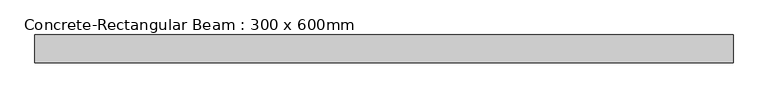
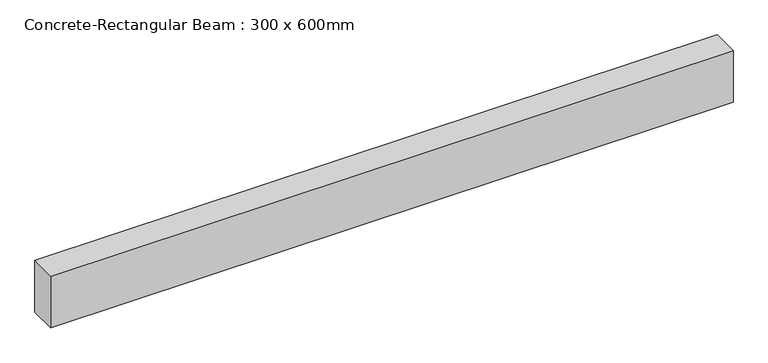
"""IFC4 building model written with IfcOpenShell, lengths in millimetres: beam geometry, Concrete-Rectangular Beam : 300 x 600mm."""

import ifcopenshell
import ifcopenshell.guid

model = None  # the IFC model being written
_history = None  # IfcOwnerHistory: only IFC2X3 demands one
_inside = {}  # id of a spatial element -> (the spatial element, [elements in it])
_under = {}  # id of a project, library or spatial element -> (it, [spatial elements below it])
_declared = {}  # id of a project -> (the project, [libraries it declares])
_typed = {}  # id of a type object -> (the type object, [elements of that type])
_made_of = {}  # id of a material, layer set ... -> (it, [elements and type objects made of it])


def new_model(schema):
    """Start an empty IFC model of exactly this schema.

    Asked for "IFC4X3", IfcOpenShell would pick the latest addendum, in which some entities
    have other attributes; the version numbers below select the first issue.
    IFC2X3 requires an IfcOwnerHistory on every rooted entity: one is made here for all.
    """
    global model, _history
    if schema == "IFC4X3":
        model = ifcopenshell.file(schema_version=(4, 3, 0, 0))
    else:
        model = ifcopenshell.file(schema=schema)
    _inside.clear()
    _under.clear()
    _declared.clear()
    _typed.clear()
    _made_of.clear()
    _history = None
    if model.schema == "IFC2X3":
        org = make("IfcOrganization", Name="unknown")
        user = make(
            "IfcPersonAndOrganization",
            ThePerson=make("IfcPerson", FamilyName="unknown"),
            TheOrganization=org,
        )
        app = make(
            "IfcApplication",
            ApplicationDeveloper=org,
            Version="unknown",
            ApplicationFullName="unknown",
            ApplicationIdentifier="unknown",
        )
        _history = make(
            "IfcOwnerHistory",
            OwningUser=user,
            OwningApplication=app,
            ChangeAction="ADDED",
            CreationDate=0,
        )
    return model


def make(cls, **values):
    """One entity of the class cls with the attributes given. An attribute that is None is left unset."""
    return model.create_entity(
        cls, **{name: value for name, value in values.items() if value is not None}
    )


def rooted(cls, **values):
    """An entity with a GlobalId (a new one), such as an element, a storey or a relation."""
    return make(cls, GlobalId=ifcopenshell.guid.new(), OwnerHistory=_history, **values)


def si_unit(unit_type, name, prefix=None):
    """IfcSIUnit, for example si_unit("LENGTHUNIT", "METRE", prefix="MILLI")."""
    return make("IfcSIUnit", UnitType=unit_type, Prefix=prefix, Name=name)


def assignment(units):
    """IfcUnitAssignment: the units of a project."""
    return None if units is None else make("IfcUnitAssignment", Units=units)


def point(xyz):
    """IfcCartesianPoint."""
    return None if xyz is None else make("IfcCartesianPoint", Coordinates=xyz)


def direction(xyz):
    """IfcDirection."""
    return None if xyz is None else make("IfcDirection", DirectionRatios=xyz)


def frame(location, z_axis=None, x_axis=None):
    """IfcAxis2Placement3D, a coordinate frame: its origin and axes. An axis left out is left unset."""
    return make(
        "IfcAxis2Placement3D",
        Location=point(location),
        Axis=direction(z_axis),
        RefDirection=direction(x_axis),
    )


def origin():
    """The frame at (0, 0, 0) with its axes left unset."""
    return frame((0.0, 0.0, 0.0))


def place(relative_to, where):
    """IfcLocalPlacement: puts the frame where relative to a parent placement (None: the world)."""
    return make(
        "IfcLocalPlacement", PlacementRelTo=relative_to, RelativePlacement=where
    )


def context(
    kind, dimensions, precision=None, world=None, true_north=None, identifier=None
):
    """IfcGeometricRepresentationContext, for example the 3D "Model" context."""
    return make(
        "IfcGeometricRepresentationContext",
        ContextIdentifier=identifier,
        ContextType=kind,
        CoordinateSpaceDimension=dimensions,
        Precision=precision,
        WorldCoordinateSystem=world,
        TrueNorth=true_north,
    )


def project(units=None, contexts=None):
    """IfcProject with its units and contexts."""
    return rooted(
        "IfcProject",
        Name="project",
        RepresentationContexts=contexts,
        UnitsInContext=assignment(units),
    )


def spatial(cls, under=None, at=None, **own):
    """A site, building, storey or space (cls), placed at a placement, below another one or the project."""
    s = rooted(cls, ObjectPlacement=at, **own)
    if under is not None:
        _under.setdefault(under.id(), (under, []))[1].append(s)
    return s


def polyline(points):
    """IfcPolyline through the points."""
    return make("IfcPolyline", Points=[point(p) for p in points])


def outline(outer, holes=None, kind="AREA"):
    """IfcArbitraryClosedProfileDef: a profile drawn as a closed curve; with holes, ...WithVoids."""
    if holes is None:
        return make("IfcArbitraryClosedProfileDef", ProfileType=kind, OuterCurve=outer)
    return make(
        "IfcArbitraryProfileDefWithVoids",
        ProfileType=kind,
        OuterCurve=outer,
        InnerCurves=holes,
    )


def extrude(swept, where, along, depth):
    """IfcExtrudedAreaSolid: the profile swept, set in the frame where, extruded along a direction by depth."""
    return make(
        "IfcExtrudedAreaSolid",
        SweptArea=swept,
        Position=where,
        ExtrudedDirection=direction(along),
        Depth=depth,
    )


def shape(context_of_items, identifier, shape_type, items):
    """IfcShapeRepresentation: the items that make up one representation, for example the "Body"."""
    return make(
        "IfcShapeRepresentation",
        ContextOfItems=context_of_items,
        RepresentationIdentifier=identifier,
        RepresentationType=shape_type,
        Items=items,
    )


def source(mapping_origin, context_of_items, identifier, shape_type, items):
    """IfcRepresentationMap: a shape defined once, which mapped items show again and again."""
    return make(
        "IfcRepresentationMap",
        MappingOrigin=mapping_origin,
        MappedRepresentation=shape(context_of_items, identifier, shape_type, items),
    )


def transform(
    local_origin,
    x_axis=None,
    y_axis=None,
    z_axis=None,
    scale=None,
    scale2=None,
    scale3=None,
    uniform=True,
):
    """IfcCartesianTransformationOperator3D, or its non-uniform kind. x_axis, y_axis, z_axis: its Axis1, 2, 3."""
    if uniform:
        return make(
            "IfcCartesianTransformationOperator3D",
            Axis1=direction(x_axis),
            Axis2=direction(y_axis),
            LocalOrigin=point(local_origin),
            Scale=scale,
            Axis3=direction(z_axis),
        )
    return make(
        "IfcCartesianTransformationOperator3DnonUniform",
        Axis1=direction(x_axis),
        Axis2=direction(y_axis),
        LocalOrigin=point(local_origin),
        Scale=scale,
        Axis3=direction(z_axis),
        Scale2=scale2,
        Scale3=scale3,
    )


def mapped(mapping_source, mapping_target):
    """IfcMappedItem: shows the shape of a source again, moved by a transform."""
    return make(
        "IfcMappedItem", MappingSource=mapping_source, MappingTarget=mapping_target
    )


def made_of(thing, what):
    """Note that an element or type object is made of a material, layer set ...; save() writes the relation."""
    if what is not None:
        _made_of.setdefault(what.id(), (what, []))[1].append(thing)
    return thing


def element(
    cls,
    number,
    at=None,
    inside=None,
    cuts=None,
    type_object=None,
    material=None,
    context=None,
    identifier="Body",
    shape_type=None,
    held_by="IfcProductDefinitionShape",
    body=None,
    shapes=None,
    **own,
):
    """One element of the class cls, such as IfcWall. Its Tag is "e" and its number.

    at: its placement. inside: the storey or other place that contains it. cuts: it is an
    opening in that element (IfcRelVoidsElement). A single representation is given by context,
    identifier, shape_type and body (its items); several are given by shapes. held_by: the class
    of the entity that holds the representations. save() writes the other relations.
    """
    e = rooted(cls, Tag="e%d" % number, ObjectPlacement=at, **own)
    if body is not None:
        shapes = [shape(context, identifier, shape_type, body)]
    if shapes is not None:
        e.Representation = make(held_by, Representations=shapes)
    if inside is not None:
        _inside.setdefault(inside.id(), (inside, []))[1].append(e)
    if cuts is not None:
        rooted(
            "IfcRelVoidsElement", RelatingBuildingElement=cuts, RelatedOpeningElement=e
        )
    if type_object is not None:
        _typed.setdefault(type_object.id(), (type_object, []))[1].append(e)
    return made_of(e, material)


def aggregate(whole, parts):
    """IfcRelAggregates: a whole, such as a stair, and the parts it consists of."""
    return rooted("IfcRelAggregates", RelatingObject=whole, RelatedObjects=parts)


def save(model, path):
    """Write the relations noted so far, then the file.

    IfcRelAggregates (storeys below a building ...), IfcRelContainedInSpatialStructure (elements
    in a storey), IfcRelDefinesByType, IfcRelAssociatesMaterial and IfcRelDeclares: one each for
    every whole, place, type object, material and project.
    """
    for whole, parts in _under.values():
        aggregate(whole, parts)
    for where, things in _inside.values():
        rooted(
            "IfcRelContainedInSpatialStructure",
            RelatedElements=things,
            RelatingStructure=where,
        )
    for kind, things in _typed.values():
        rooted("IfcRelDefinesByType", RelatedObjects=things, RelatingType=kind)
    for what, things in _made_of.values():
        rooted("IfcRelAssociatesMaterial", RelatedObjects=things, RelatingMaterial=what)
    for by, libraries in _declared.values():
        rooted("IfcRelDeclares", RelatingContext=by, RelatedDefinitions=libraries)
    model.write(path)


def concrete_rectangular_beam_300_x_600mm_b31908cc(model_context):
    return source(origin(), model_context, "Body", "SweptSolid", [
        extrude(outline(polyline([(3750.0, 150.0), (3750.0, -150.0), (-3750.0, -150.0), (-3750.0, 150.0), (3750.0, 150.0)])), frame((0.0, 0.0, -300.0), z_axis=(0.0, 0.0, 1.0), x_axis=(1.0, 0.0, 0.0)), (0.0, 0.0, 1.0), 600.0),
    ])


if __name__ == "__main__":
    model = new_model("IFC4")
    model_context = context("Model", 3, world=origin())
    ifc_project = project(units=[si_unit("LENGTHUNIT", "METRE", prefix="MILLI")], contexts=[model_context])
    site = spatial("IfcSite", under=ifc_project)
    building = spatial("IfcBuilding", under=site)
    placement = place(None, origin())
    concrete_rectangular_beam_300_x_600mm_shape = concrete_rectangular_beam_300_x_600mm_b31908cc(model_context)
    element("IfcBeam", 1, ObjectType="Concrete-Rectangular Beam : 300 x 600mm", at=placement, inside=building, context=model_context, shape_type="MappedRepresentation", body=[
        mapped(concrete_rectangular_beam_300_x_600mm_shape, transform((0.0, 0.0, 0.0), x_axis=(1.0, 0.0, 0.0), y_axis=(0.0, 1.0, 0.0), z_axis=(0.0, 0.0, 1.0))),
    ])
    save(model, "model.ifc")

# Revit data of these elements
# Type "Concrete-Rectangular Beam : 300 x 600mm"
#   Length [instance default] = 1524 mm
#   b = 300 mm
#   h = 600 mm
#   Structural Material [instance default] = Concrete, Cast-in-Place gray
#   Assembly Code = ""
# Element 1 (IfcBeam, "Concrete-Rectangular Beam : 300 x 600mm")
#   Materials on its faces: "Concrete, Cast-in-Place gray"
# Materials
#   "Concrete, Cast-in-Place gray": class "Concrete", colour RGB 192 192 192, transparency 0, Description = "Cast-in-place concrete", Cost = 0
